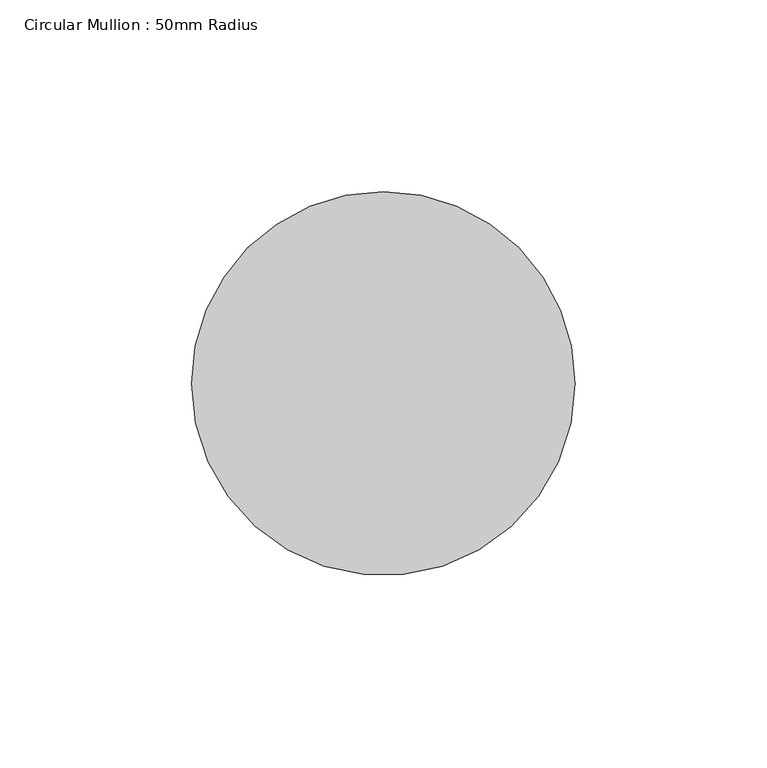
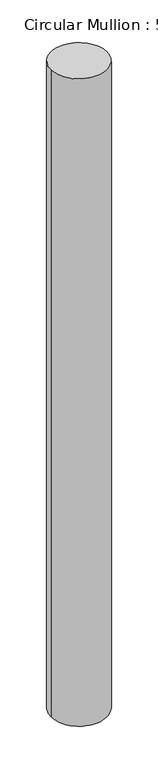
"""IFC4 building model written with IfcOpenShell, lengths in millimetres: member geometry, Circular Mullion : 50mm Radius."""

from ifc_helpers import new_model, si_unit, frame, origin, place, context, project, spatial, ellipse_curve, source, transform, mapped, element, save
from ifc_brep_helpers import plane_surface, cylinder_surface, advanced_brep


def circular_mullion_50mm_radius_74ae809d(model_context):
    return source(origin(), model_context, "Body", "AdvancedBrep", [
        advanced_brep(
        [(-100.0, 0.0, 0.8215301), (0.0, 0.0, 0.0), (0.0, 0.0, -1216.5670082), (-100.0, 0.0, -1217.440251)],
        [
            (0, 1, ellipse_curve(frame((-50.0, 0.0, 0.410765), z_axis=(-0.008213641473767847, -0.018343770086312706, -0.9997980006945207), x_axis=(-0.4085827271229978, -0.9124999711175309, 0.020098701630680983)), 50.010102, 50.0)),
            (1, 2),
            (2, 3, ellipse_curve(frame((-50.0, 0.0, -1217.0036296), z_axis=(-0.008730435122154458, -0.01949794073015418, 0.9997717788624869), x_axis=(0.40857201117075964, 0.9124760388622499, 0.021363290714174542)), 50.0114137, 50.0)),
            (3, 0),
            (1, 0, ellipse_curve(frame((-50.0, 0.0, 0.410765), z_axis=(-0.008213641473767847, -0.018343770086312706, -0.9997980006945207), x_axis=(-0.4085827271229978, -0.9124999711175309, 0.020098701630680983)), 50.010102, 50.0)),
            (3, 2, ellipse_curve(frame((-50.0, 0.0, -1217.0036296), z_axis=(-0.008730435122154458, -0.01949794073015418, 0.9997717788624869), x_axis=(0.40857201117075964, 0.9124760388622499, 0.021363290714174542)), 50.0114137, 50.0)),
        ],
        [
            cylinder_surface(frame((-50.0, 0.0, 0.0), z_axis=(0.0, 0.0, 1.0), x_axis=(1.0, 0.0, 0.0)), 50.0),
            plane_surface(frame((-278.1861846, 124.5611765, 0.0), z_axis=(0.008213641473767849, 0.01834377008631271, 0.999798000694521), x_axis=(0.40858272712299926, 0.9124999711175303, -0.020098701630680033))),
            plane_surface(frame((-278.1861846, 124.5611765, -1216.5670082), z_axis=(0.008730435122154458, 0.01949794073015418, -0.9997717788624869), x_axis=(0.40857201117075975, 0.9124760388622498, 0.021363290714184306))),
        ],
        [
            (0, [[1, 2, 3, 4]]),
            (0, [[5, -4, 6, -2]]),
            (1, [[-1, -5]]),
            (2, [[-6, -3]]),
        ],
    ),
    ])


if __name__ == "__main__":
    model = new_model("IFC4")
    model_context = context("Model", 3, world=origin())
    ifc_project = project(units=[si_unit("LENGTHUNIT", "METRE", prefix="MILLI")], contexts=[model_context])
    site = spatial("IfcSite", under=ifc_project)
    building = spatial("IfcBuilding", under=site)
    placement = place(None, origin())
    circular_mullion_50mm_radius_shape = circular_mullion_50mm_radius_74ae809d(model_context)
    element("IfcMember", 1, ObjectType="Circular Mullion : 50mm Radius", at=placement, inside=building, context=model_context, shape_type="MappedRepresentation", body=[
        mapped(circular_mullion_50mm_radius_shape, transform((0.0, 0.0, 0.0), x_axis=(1.0, 0.0, 0.0), y_axis=(0.0, 1.0, 0.0), z_axis=(0.0, 0.0, 1.0))),
    ])
    save(model, "model.ifc")

# Revit data of these elements
# Type "Circular Mullion : 50mm Radius"
#   built-in parameter 1007350 = 0.164042 (stored number, unit not read)
# Element 1 (IfcMember, "Circular Mullion : 50mm Radius")
#   Materials on its faces: "Aluminium"
# Materials
#   "Aluminium": class "Metal", colour RGB 247 247 247, transparency 0, Description = "Aluminium 6061", Cost = 0
